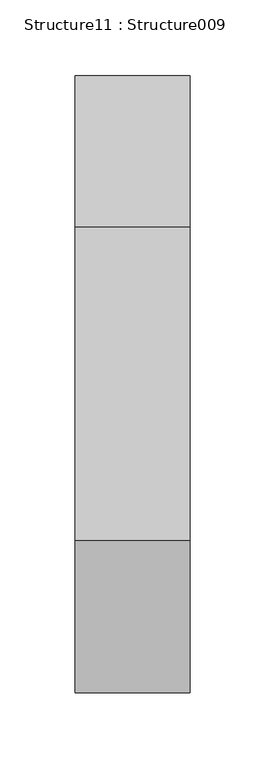
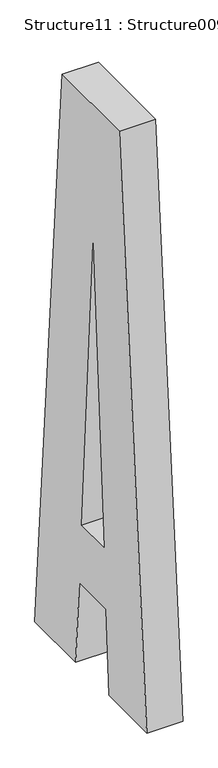
"""IFC4 building model written with IfcOpenShell, lengths in millimetres: proxy geometry, Structure11 : Structure009."""

from ifc_helpers import new_model, si_unit, frame, origin, place, context, project, spatial, polyline, outline, extrude, source, transform, mapped, element, save


def structure11_structure009_49891c69(model_context):
    return source(origin(), model_context, "Body", "SweptSolid", [
        extrude(outline(polyline([(139.0265423, 0.0), (38.4204791, -1280.4310236), (-170.1112862, -1280.4310236), (-270.7046417, 0.0), (-120.7291397, 0.0), (-107.9113, -184.732773), (-10.9565843, -184.732773), (0.0, 0.0), (139.0265423, 0.0)]), holes=[polyline([(-18.2838478, -318.2763636), (-100.5933555, -318.2763636), (-58.5333894, -971.316069), (-18.2838478, -318.2763636)])]), frame((-35624.0862846, 275588.4150451, 4479.6663888), z_axis=(1.0, 0.0, 1.354250045437766e-12), x_axis=(0.0, -1.0, 0.0)), (0.0, 0.0, 1.0), 76.2),
    ])


if __name__ == "__main__":
    model = new_model("IFC4")
    model_context = context("Model", 3, world=origin())
    ifc_project = project(units=[si_unit("LENGTHUNIT", "METRE", prefix="MILLI")], contexts=[model_context])
    site = spatial("IfcSite", under=ifc_project)
    building = spatial("IfcBuilding", under=site)
    placement = place(None, origin())
    structure11_structure009_shape = structure11_structure009_49891c69(model_context)
    element("IfcBuildingElementProxy", 1, Name="Structure11 : Structure009", ObjectType="Structure11 : Structure009", at=placement, inside=building, context=model_context, shape_type="MappedRepresentation", body=[
        mapped(structure11_structure009_shape, transform((0.0, 0.0, 0.0), x_axis=(1.0, 0.0, 0.0), y_axis=(0.0, 1.0, 0.0), z_axis=(0.0, 0.0, 1.0))),
    ])
    save(model, "model.ifc")

# Revit data of these elements
# Type "Structure11 : Structure009"
#   NameOverride = "Structure009"
# Element 1 (IfcBuildingElementProxy, "Structure11 : Structure009")
#   Materials on its faces: "BRUSHED ALUMINUM LETTERING"
# Materials
#   "BRUSHED ALUMINUM LETTERING": class "Unassigned", colour RGB 169 181 186, transparency 0, Cost = 0
